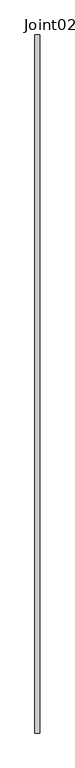
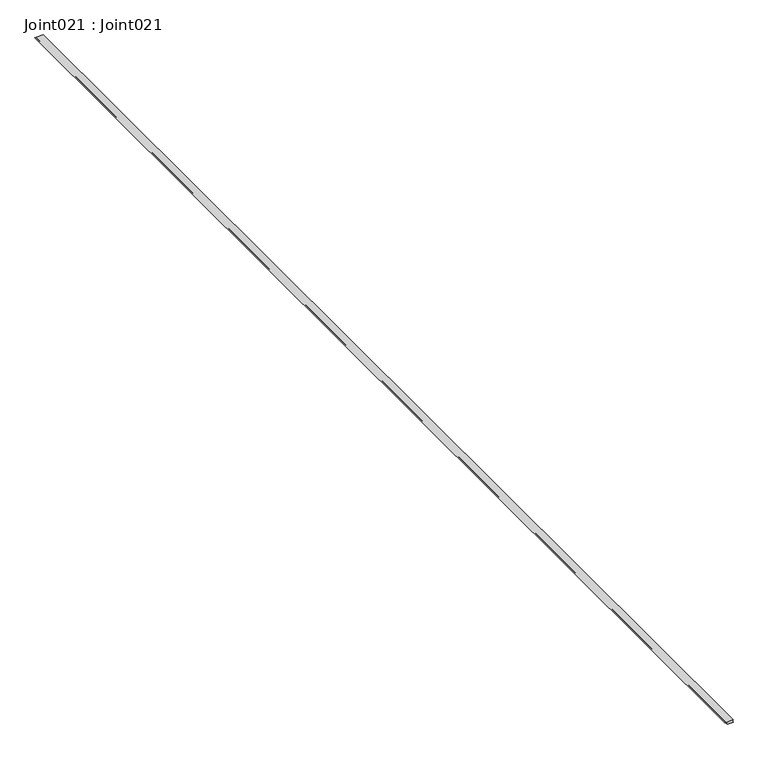
"""IFC4 building model written with IfcOpenShell, lengths in millimetres: proxy geometry, Joint021 : Joint021."""

from ifc_helpers import new_model, si_unit, point, frame, frame_2d, origin, place, context, project, spatial, polyline, circle_curve, trimmed, segment, composite_curve, outline, extrude, source, transform, mapped, element, save


def joint021_joint021_d57ccf5f(model_context):
    return source(origin(), model_context, "Body", "SweptSolid", [
        extrude(outline(composite_curve([segment(polyline([(42101.1735582, -1091.7086898), (42101.1735582, -1105.5567407)]), True, "CONTINUOUS"), segment(trimmed(circle_curve(frame_2d((42094.9766062, -1107.8918285)), 6.6222994), [point((42101.1735582, -1105.5567407))], [point((42096.9562501, -1101.572346))], True, "CARTESIAN"), True, "CONTINUOUS"), segment(polyline([(42096.9562501, -1101.572346), (42096.9562501, -1091.7086898)]), True, "CONTINUOUS"), segment(trimmed(circle_curve(frame_2d((42099.0649041, -1083.7985335)), 8.1863908), [point((42096.9562501, -1091.7086898))], [point((42101.1735582, -1091.7086898))], True, "CARTESIAN"), True, "CONTINUOUS")], self_intersect=False)), frame((0.0, -1052.8906574, 0.0), z_axis=(0.0, 1.0, 0.0), x_axis=(0.0, 0.0, 1.0)), (0.0, 0.0, 1.0), 2000.0),
    ])


if __name__ == "__main__":
    model = new_model("IFC4")
    model_context = context("Model", 3, world=origin())
    ifc_project = project(units=[si_unit("LENGTHUNIT", "METRE", prefix="MILLI")], contexts=[model_context])
    site = spatial("IfcSite", under=ifc_project)
    building = spatial("IfcBuilding", under=site)
    placement = place(None, origin())
    joint021_joint021_shape = joint021_joint021_d57ccf5f(model_context)
    element("IfcBuildingElementProxy", 1, Name="Joint021 : Joint021", ObjectType="Joint021 : Joint021", at=placement, inside=building, context=model_context, shape_type="MappedRepresentation", body=[
        mapped(joint021_joint021_shape, transform((0.0, 0.0, 0.0), x_axis=(1.0, 0.0, 0.0), y_axis=(0.0, 1.0, 0.0), z_axis=(0.0, 0.0, 1.0))),
    ])
    save(model, "model.ifc")

# Revit data of these elements
# Type "Joint021 : Joint021"
#   NameOverride = "Joint021"
# Element 1 (IfcBuildingElementProxy, "Joint021 : Joint021")
#   Materials on its faces: "SEALANT"
# Materials
#   "SEALANT": class "Unassigned", colour RGB 142 225 148, transparency 0
